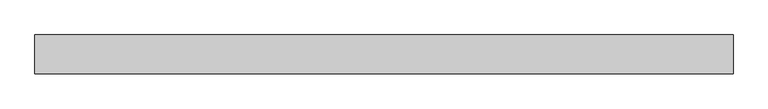
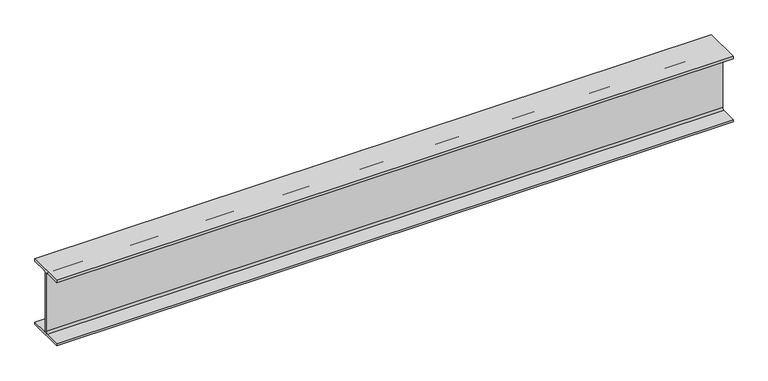
"""IFC4 building model written with IfcOpenShell, lengths in millimetres: beam geometry, Old_Steel Beam_H-KSD3502 : H_SB_ASB_H-200×200x8x12."""

from ifc_helpers import new_model, si_unit, point, frame, frame_2d, origin, place, context, project, spatial, polyline, circle_curve, trimmed, segment, composite_curve, outline, extrude, source, transform, mapped, element, save


def beam_fd5dc25f(model_context):
    return source(origin(), model_context, "Body", "SweptSolid", [
        extrude(outline(composite_curve([segment(polyline([(82.5, -141.5), (82.5, -151.7), (-82.5, -151.7), (-82.5, -141.5), (-11.9, -141.5)]), True, "CONTINUOUS"), segment(trimmed(circle_curve(frame_2d((-11.9, -132.6)), 8.9), [point((-11.9, -141.5))], [point((-3.0, -132.6))], True, "CARTESIAN"), True, "CONTINUOUS"), segment(polyline([(-3.0, -132.6), (-3.0, 132.6)]), True, "CONTINUOUS"), segment(trimmed(circle_curve(frame_2d((-11.9, 132.6)), 8.9), [point((-3.0, 132.6))], [point((-11.9, 141.5))], True, "CARTESIAN"), True, "CONTINUOUS"), segment(polyline([(-11.9, 141.5), (-82.5, 141.5), (-82.5, 151.7), (82.5, 151.7), (82.5, 141.5), (11.9, 141.5)]), True, "CONTINUOUS"), segment(trimmed(circle_curve(frame_2d((11.9, 132.6)), 8.9), [point((11.9, 141.5))], [point((3.0, 132.6))], True, "CARTESIAN"), True, "CONTINUOUS"), segment(polyline([(3.0, 132.6), (3.0, -132.6)]), True, "CONTINUOUS"), segment(trimmed(circle_curve(frame_2d((11.9, -132.6)), 8.9), [point((3.0, -132.6))], [point((11.9, -141.5))], True, "CARTESIAN"), True, "CONTINUOUS"), segment(polyline([(11.9, -141.5), (82.5, -141.5)]), True, "CONTINUOUS")], self_intersect=False)), frame((-1273.3895071, 0.0, 0.0), z_axis=(1.0, 0.0, 0.0), x_axis=(0.0, 1.0, 0.0)), (0.0, 0.0, 1.0), 2971.0125575),
    ])


if __name__ == "__main__":
    model = new_model("IFC4")
    model_context = context("Model", 3, world=origin())
    ifc_project = project(units=[si_unit("LENGTHUNIT", "METRE", prefix="MILLI")], contexts=[model_context])
    site = spatial("IfcSite", under=ifc_project)
    building = spatial("IfcBuilding", under=site)
    placement = place(None, origin())
    beam_shape = beam_fd5dc25f(model_context)
    element("IfcBeam", 1, ObjectType="Old_Steel Beam_H-KSD3502 : H_SB_ASB_H-200×200x8x12", at=placement, inside=building, context=model_context, shape_type="MappedRepresentation", body=[
        mapped(beam_shape, transform((0.0, 0.0, 0.0), x_axis=(1.0, 0.0, 0.0), y_axis=(0.0, 1.0, 0.0), z_axis=(0.0, 0.0, 1.0))),
    ])
    save(model, "model.ifc")

# Revit data of these elements
# Type "Old_Steel Beam_H-KSD3502 : H_SB_ASB_H-200×200x8x12"
#   Width = 20.0 cm
#   Web Thickness = 0.8 cm
#   Web Fillet = 1.3 cm
#   Warping Constant = 141376.0 cm⁶
#   Torsional Moment of Inertia = 26.2485 cm⁴
#   Torsional Modulus = 1.0 cm³
#   Section Area = 63.53 cm²
#   Plastic Modulus weak axis = 244.0 cm³
#   Plastic Modulus strong axis = 525.0 cm³
#   Perimeter = 1.16 m²/m
#   Nominal Weight = 49.90 kgf/m
#   Moment of Inertia weak axis = 1600.00 cm⁴
#   Moment of Inertia strong axis = 4720.00 cm⁴
#   Height = 20.0 cm
#   Flange Thickness = 1.2 cm
#   Elastic Modulus weak axis = 160.0 cm³
#   Elastic Modulus strong axis = 472.0 cm³
#   Centroid Vertical = 10.0 cm
#   Centroid Horizontal = 10.0 cm
#   Length [instance default] = 1.5240 m
#   Structural Material [instance default] = Steel, 45-345
#   Assembly Code = ""
# Element 1 (IfcBeam, "Old_Steel Beam_H-KSD3502 : H_SB_ASB_H-200×200x8x12")
#   Structural Material = none
# Materials
#   "Steel, 45-345": class "Metal", colour RGB 189 187 185, transparency 0, Description = "Steel 345 MPa", Cost = 0
